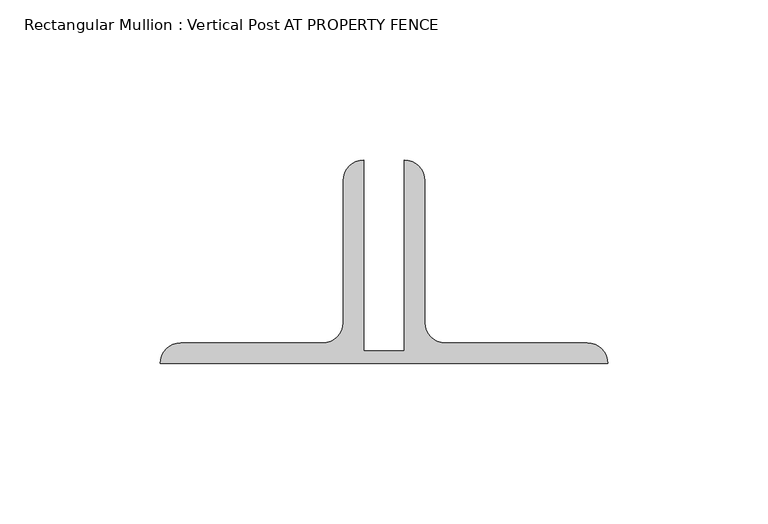
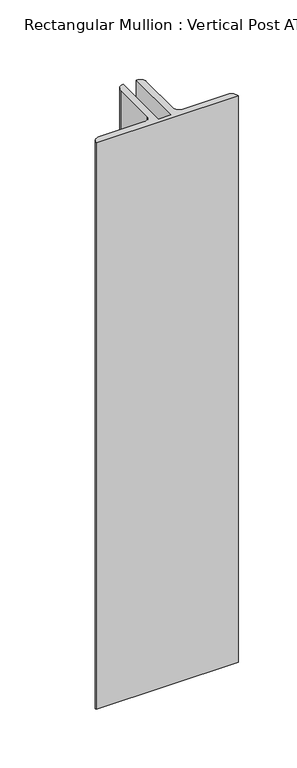
"""IFC4 building model written with IfcOpenShell, lengths in millimetres: member geometry, Rectangular Mullion : Vertical Post AT PROPERTY FENCE."""

from ifc_helpers import new_model, si_unit, point, frame, frame_2d, origin, place, context, project, spatial, polyline, circle_curve, trimmed, segment, composite_curve, outline, extrude, source, transform, mapped, element, save


def rectangular_mullion_vertical_post_at_property_fence_bad6d568(model_context):
    return source(origin(), model_context, "Body", "SweptSolid", [
        extrude(outline(composite_curve([segment(polyline([(-63.5, 22.9145205), (-63.5, 82.55)]), True, "CONTINUOUS"), segment(trimmed(circle_curve(frame_2d((-63.5, 76.2)), 6.35), [point((-63.5, 82.55))], [point((-57.15, 76.2))], False, "CARTESIAN"), True, "CONTINUOUS"), segment(polyline([(-57.15, 76.2), (-57.15, 31.75)]), True, "CONTINUOUS"), segment(trimmed(circle_curve(frame_2d((-50.8, 31.75)), 6.35), [point((-57.15, 31.75))], [point((-50.8, 25.4))], True, "CARTESIAN"), True, "CONTINUOUS"), segment(polyline([(-50.8, 25.4), (-6.35, 25.4)]), True, "CONTINUOUS"), segment(trimmed(circle_curve(frame_2d((-6.35, 19.05)), 6.35), [point((-6.35, 25.4))], [point((0.0, 19.05))], False, "CARTESIAN"), True, "CONTINUOUS"), segment(polyline([(0.0, 19.05), (-139.7, 19.05)]), True, "CONTINUOUS"), segment(trimmed(circle_curve(frame_2d((-133.35, 19.05)), 6.35), [point((-139.7, 19.05))], [point((-133.35, 25.4))], False, "CARTESIAN"), True, "CONTINUOUS"), segment(polyline([(-133.35, 25.4), (-88.9, 25.4)]), True, "CONTINUOUS"), segment(trimmed(circle_curve(frame_2d((-88.9, 31.75)), 6.35), [point((-88.9, 25.4))], [point((-82.55, 31.75))], True, "CARTESIAN"), True, "CONTINUOUS"), segment(polyline([(-82.55, 31.75), (-82.55, 76.2)]), True, "CONTINUOUS"), segment(trimmed(circle_curve(frame_2d((-76.2, 76.2)), 6.35), [point((-82.55, 76.2))], [point((-76.2, 82.55))], False, "CARTESIAN"), True, "CONTINUOUS"), segment(polyline([(-76.2, 82.55), (-76.2, 22.9145205), (-63.5, 22.9145205)]), True, "CONTINUOUS")], self_intersect=False)), frame((0.0, 0.0, -588.8534967), z_axis=(0.0, 0.0, 1.0), x_axis=(1.0, 0.0, 0.0)), (0.0, 0.0, 1.0), 588.8534967),
    ])


if __name__ == "__main__":
    model = new_model("IFC4")
    model_context = context("Model", 3, world=origin())
    ifc_project = project(units=[si_unit("LENGTHUNIT", "METRE", prefix="MILLI")], contexts=[model_context])
    site = spatial("IfcSite", under=ifc_project)
    building = spatial("IfcBuilding", under=site)
    placement = place(None, origin())
    rectangular_mullion_vertical_post_at_property_fence_shape = rectangular_mullion_vertical_post_at_property_fence_bad6d568(model_context)
    element("IfcMember", 1, ObjectType="Rectangular Mullion : Vertical Post AT PROPERTY FENCE", at=placement, inside=building, context=model_context, shape_type="MappedRepresentation", body=[
        mapped(rectangular_mullion_vertical_post_at_property_fence_shape, transform((0.0, 0.0, 0.0), x_axis=(1.0, 0.0, 0.0), y_axis=(0.0, 1.0, 0.0), z_axis=(0.0, 0.0, 1.0))),
    ])
    save(model, "model.ifc")

# Revit data of these elements
# Type "Rectangular Mullion : Vertical Post AT PROPERTY FENCE"
#   built-in parameter 1007351 = -0.0625 (stored number, unit not read)
#   built-in parameter 1007322 = 0.0126789 (stored number, unit not read)
#   built-in parameter 1007321 = 0.229167 (stored number, unit not read)
#   built-in parameter 1007320 = 0.229167 (stored number, unit not read)
# Element 1 (IfcMember, "Rectangular Mullion : Vertical Post AT PROPERTY FENCE")
#   Materials on its faces: "MAIN FENCE POST: (2) BACK/BACK GALVANIZED ANGLES (2) L2 1/2 X 2 1/2 X 1/4\") ANCHORED TO 8\"W X 42\" DEEP CONCRETE FOOTING(1)"
# Materials
#   "MAIN FENCE POST: (2) BACK/BACK GALVANIZED ANGLES (2) L2 1/2 X 2 1/2 X 1/4\") ANCHORED TO 8\"W X 42\" DEEP CONCRETE FOOTING(1)": class "Unassigned", colour RGB 211 211 211, transparency 0, Cost = 0
